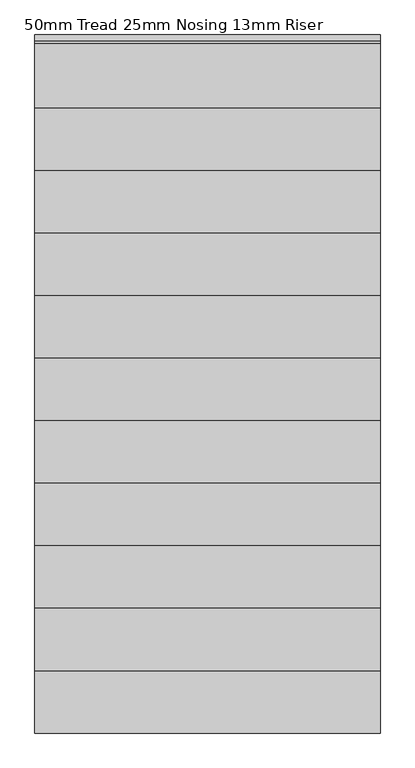
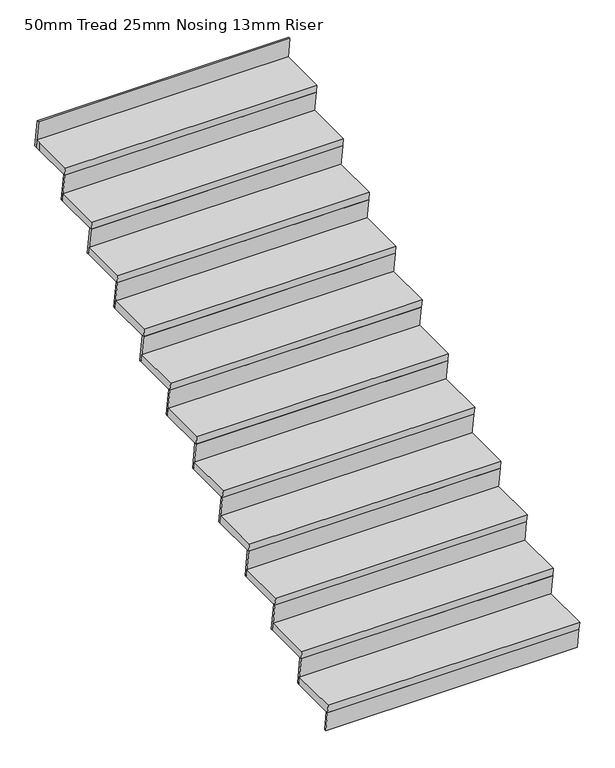
"""IFC4 building model written with IfcOpenShell, lengths in millimetres: stair flight geometry, 50mm Tread 25mm Nosing 13mm Riser."""

from ifc_helpers import new_model, si_unit, origin, place, context, project, spatial, faceted_brep, source, transform, mapped, element, save


def stair_flight_50mm_tread_25mm_nosing_13mm_riser_20ac8c47(model_context):
    return source(origin(), model_context, "Body", "Brep", [
        faceted_brep([(-499.4393676, 4584.7509075, 12676.4705882), (-499.4393676, 4591.8342409, 12626.4705882), (-2019.4393676, 4591.8342409, 12626.4705882), (-2019.4393676, 4584.7509075, 12676.4705882), (-2019.4393676, 4284.7509075, 12676.4705882), (-499.4393676, 4284.7509075, 12676.4705882), (-499.4393676, 4291.8342409, 12626.4705882), (-2019.4393676, 4291.8342409, 12626.4705882)], [[[0, 1, 2, 3]], [[3, 4, 5, 0]], [[2, 1, 6, 7]], [[4, 3, 2, 7]], [[0, 5, 6, 1]], [[5, 4, 7, 6]]]),
        faceted_brep([(-499.4393676, 4291.8342409, 12626.4705882), (-499.4393676, 4309.7509075, 12500.0), (-499.4393676, 4322.3757185, 12500.0), (-499.4393676, 4304.4590518, 12626.4705882), (-2019.4393676, 4291.8342409, 12626.4705882), (-2019.4393676, 4304.4590518, 12626.4705882), (-2019.4393676, 4322.3757185, 12500.0), (-2019.4393676, 4309.7509075, 12500.0)], [[[0, 1, 2, 3]], [[4, 5, 6, 7]], [[1, 0, 4, 7]], [[2, 1, 7, 6]], [[3, 2, 6, 5]], [[0, 3, 5, 4]]]),
        faceted_brep([(-499.4393676, 4566.8342409, 12802.9411765), (-499.4393676, 4591.8342409, 12626.4705882), (-499.4393676, 4604.4590518, 12626.4705882), (-499.4393676, 4579.4590518, 12802.9411765), (-2019.4393676, 4566.8342409, 12802.9411765), (-2019.4393676, 4579.4590518, 12802.9411765), (-2019.4393676, 4604.4590518, 12626.4705882), (-2019.4393676, 4591.8342409, 12626.4705882)], [[[0, 1, 2, 3]], [[4, 5, 6, 7]], [[1, 0, 4, 7]], [[2, 1, 7, 6]], [[3, 2, 6, 5]], [[0, 3, 5, 4]]]),
        faceted_brep([(-2019.4393676, 4859.7509075, 12852.9411765), (-2019.4393676, 4559.7509075, 12852.9411765), (-499.4393676, 4559.7509075, 12852.9411765), (-499.4393676, 4859.7509075, 12852.9411765), (-2019.4393676, 4866.8342409, 12802.9411765), (-499.4393676, 4866.8342409, 12802.9411765), (-499.4393676, 4566.8342409, 12802.9411765), (-2019.4393676, 4566.8342409, 12802.9411765)], [[[0, 1, 2, 3]], [[4, 5, 6, 7]], [[1, 0, 4, 7]], [[3, 2, 6, 5]], [[3, 5, 4, 0]], [[2, 1, 7, 6]]]),
        faceted_brep([(-499.4393676, 4841.8342409, 12979.4117647), (-499.4393676, 4866.8342409, 12802.9411765), (-499.4393676, 4879.4590518, 12802.9411765), (-499.4393676, 4854.4590518, 12979.4117647), (-2019.4393676, 4841.8342409, 12979.4117647), (-2019.4393676, 4854.4590518, 12979.4117647), (-2019.4393676, 4879.4590518, 12802.9411765), (-2019.4393676, 4866.8342409, 12802.9411765)], [[[0, 1, 2, 3]], [[4, 5, 6, 7]], [[1, 0, 4, 7]], [[2, 1, 7, 6]], [[3, 2, 6, 5]], [[0, 3, 5, 4]]]),
        faceted_brep([(-2019.4393676, 5134.7509075, 13029.4117647), (-2019.4393676, 4834.7509075, 13029.4117647), (-499.4393676, 4834.7509075, 13029.4117647), (-499.4393676, 5134.7509075, 13029.4117647), (-2019.4393676, 5141.8342409, 12979.4117647), (-499.4393676, 5141.8342409, 12979.4117647), (-499.4393676, 4841.8342409, 12979.4117647), (-2019.4393676, 4841.8342409, 12979.4117647)], [[[0, 1, 2, 3]], [[4, 5, 6, 7]], [[1, 0, 4, 7]], [[3, 2, 6, 5]], [[3, 5, 4, 0]], [[2, 1, 7, 6]]]),
        faceted_brep([(-499.4393676, 5116.8342409, 13155.8823529), (-499.4393676, 5141.8342409, 12979.4117647), (-499.4393676, 5154.4590518, 12979.4117647), (-499.4393676, 5129.4590518, 13155.8823529), (-2019.4393676, 5116.8342409, 13155.8823529), (-2019.4393676, 5129.4590518, 13155.8823529), (-2019.4393676, 5154.4590518, 12979.4117647), (-2019.4393676, 5141.8342409, 12979.4117647)], [[[0, 1, 2, 3]], [[4, 5, 6, 7]], [[1, 0, 4, 7]], [[2, 1, 7, 6]], [[3, 2, 6, 5]], [[0, 3, 5, 4]]]),
        faceted_brep([(-2019.4393676, 5409.7509075, 13205.8823529), (-2019.4393676, 5109.7509075, 13205.8823529), (-499.4393676, 5109.7509075, 13205.8823529), (-499.4393676, 5409.7509075, 13205.8823529), (-2019.4393676, 5416.8342409, 13155.8823529), (-499.4393676, 5416.8342409, 13155.8823529), (-499.4393676, 5116.8342409, 13155.8823529), (-2019.4393676, 5116.8342409, 13155.8823529)], [[[0, 1, 2, 3]], [[4, 5, 6, 7]], [[1, 0, 4, 7]], [[3, 2, 6, 5]], [[3, 5, 4, 0]], [[2, 1, 7, 6]]]),
        faceted_brep([(-499.4393676, 5391.8342409, 13332.3529412), (-499.4393676, 5416.8342409, 13155.8823529), (-499.4393676, 5429.4590518, 13155.8823529), (-499.4393676, 5404.4590518, 13332.3529412), (-2019.4393676, 5391.8342409, 13332.3529412), (-2019.4393676, 5404.4590518, 13332.3529412), (-2019.4393676, 5429.4590518, 13155.8823529), (-2019.4393676, 5416.8342409, 13155.8823529)], [[[0, 1, 2, 3]], [[4, 5, 6, 7]], [[1, 0, 4, 7]], [[2, 1, 7, 6]], [[3, 2, 6, 5]], [[0, 3, 5, 4]]]),
        faceted_brep([(-2019.4393676, 5684.7509075, 13382.3529412), (-2019.4393676, 5384.7509075, 13382.3529412), (-499.4393676, 5384.7509075, 13382.3529412), (-499.4393676, 5684.7509075, 13382.3529412), (-2019.4393676, 5691.8342409, 13332.3529412), (-499.4393676, 5691.8342409, 13332.3529412), (-499.4393676, 5391.8342409, 13332.3529412), (-2019.4393676, 5391.8342409, 13332.3529412)], [[[0, 1, 2, 3]], [[4, 5, 6, 7]], [[1, 0, 4, 7]], [[3, 2, 6, 5]], [[3, 5, 4, 0]], [[2, 1, 7, 6]]]),
        faceted_brep([(-499.4393676, 5666.8342409, 13508.8235294), (-499.4393676, 5691.8342409, 13332.3529412), (-499.4393676, 5704.4590518, 13332.3529412), (-499.4393676, 5679.4590518, 13508.8235294), (-2019.4393676, 5666.8342409, 13508.8235294), (-2019.4393676, 5679.4590518, 13508.8235294), (-2019.4393676, 5704.4590518, 13332.3529412), (-2019.4393676, 5691.8342409, 13332.3529412)], [[[0, 1, 2, 3]], [[4, 5, 6, 7]], [[1, 0, 4, 7]], [[2, 1, 7, 6]], [[3, 2, 6, 5]], [[0, 3, 5, 4]]]),
        faceted_brep([(-2019.4393676, 5959.7509075, 13558.8235294), (-2019.4393676, 5659.7509075, 13558.8235294), (-499.4393676, 5659.7509075, 13558.8235294), (-499.4393676, 5959.7509075, 13558.8235294), (-2019.4393676, 5966.8342409, 13508.8235294), (-499.4393676, 5966.8342409, 13508.8235294), (-499.4393676, 5666.8342409, 13508.8235294), (-2019.4393676, 5666.8342409, 13508.8235294)], [[[0, 1, 2, 3]], [[4, 5, 6, 7]], [[1, 0, 4, 7]], [[3, 2, 6, 5]], [[3, 5, 4, 0]], [[2, 1, 7, 6]]]),
        faceted_brep([(-499.4393676, 5941.8342409, 13685.2941176), (-499.4393676, 5966.8342409, 13508.8235294), (-499.4393676, 5979.4590518, 13508.8235294), (-499.4393676, 5954.4590518, 13685.2941176), (-2019.4393676, 5941.8342409, 13685.2941176), (-2019.4393676, 5954.4590518, 13685.2941176), (-2019.4393676, 5979.4590518, 13508.8235294), (-2019.4393676, 5966.8342409, 13508.8235294)], [[[0, 1, 2, 3]], [[4, 5, 6, 7]], [[1, 0, 4, 7]], [[2, 1, 7, 6]], [[3, 2, 6, 5]], [[0, 3, 5, 4]]]),
        faceted_brep([(-2019.4393676, 6234.7509075, 13735.2941176), (-2019.4393676, 5934.7509075, 13735.2941176), (-499.4393676, 5934.7509075, 13735.2941176), (-499.4393676, 6234.7509075, 13735.2941176), (-2019.4393676, 6241.8342409, 13685.2941176), (-499.4393676, 6241.8342409, 13685.2941176), (-499.4393676, 5941.8342409, 13685.2941176), (-2019.4393676, 5941.8342409, 13685.2941176)], [[[0, 1, 2, 3]], [[4, 5, 6, 7]], [[1, 0, 4, 7]], [[3, 2, 6, 5]], [[3, 5, 4, 0]], [[2, 1, 7, 6]]]),
        faceted_brep([(-499.4393676, 6216.8342409, 13861.7647059), (-499.4393676, 6241.8342409, 13685.2941176), (-499.4393676, 6254.4590518, 13685.2941176), (-499.4393676, 6229.4590518, 13861.7647059), (-2019.4393676, 6216.8342409, 13861.7647059), (-2019.4393676, 6229.4590518, 13861.7647059), (-2019.4393676, 6254.4590518, 13685.2941176), (-2019.4393676, 6241.8342409, 13685.2941176)], [[[0, 1, 2, 3]], [[4, 5, 6, 7]], [[1, 0, 4, 7]], [[2, 1, 7, 6]], [[3, 2, 6, 5]], [[0, 3, 5, 4]]]),
        faceted_brep([(-2019.4393676, 6509.7509075, 13911.7647059), (-2019.4393676, 6209.7509075, 13911.7647059), (-499.4393676, 6209.7509075, 13911.7647059), (-499.4393676, 6509.7509075, 13911.7647059), (-2019.4393676, 6516.8342409, 13861.7647059), (-499.4393676, 6516.8342409, 13861.7647059), (-499.4393676, 6216.8342409, 13861.7647059), (-2019.4393676, 6216.8342409, 13861.7647059)], [[[0, 1, 2, 3]], [[4, 5, 6, 7]], [[1, 0, 4, 7]], [[3, 2, 6, 5]], [[3, 5, 4, 0]], [[2, 1, 7, 6]]]),
        faceted_brep([(-499.4393676, 6491.8342409, 14038.2352941), (-499.4393676, 6516.8342409, 13861.7647059), (-499.4393676, 6529.4590518, 13861.7647059), (-499.4393676, 6504.4590518, 14038.2352941), (-2019.4393676, 6491.8342409, 14038.2352941), (-2019.4393676, 6504.4590518, 14038.2352941), (-2019.4393676, 6529.4590518, 13861.7647059), (-2019.4393676, 6516.8342409, 13861.7647059)], [[[0, 1, 2, 3]], [[4, 5, 6, 7]], [[1, 0, 4, 7]], [[2, 1, 7, 6]], [[3, 2, 6, 5]], [[0, 3, 5, 4]]]),
        faceted_brep([(-2019.4393676, 6784.7509075, 14088.2352941), (-2019.4393676, 6484.7509075, 14088.2352941), (-499.4393676, 6484.7509075, 14088.2352941), (-499.4393676, 6784.7509075, 14088.2352941), (-2019.4393676, 6791.8342409, 14038.2352941), (-499.4393676, 6791.8342409, 14038.2352941), (-499.4393676, 6491.8342409, 14038.2352941), (-2019.4393676, 6491.8342409, 14038.2352941)], [[[0, 1, 2, 3]], [[4, 5, 6, 7]], [[1, 0, 4, 7]], [[3, 2, 6, 5]], [[3, 5, 4, 0]], [[2, 1, 7, 6]]]),
        faceted_brep([(-499.4393676, 6766.8342409, 14214.7058824), (-499.4393676, 6791.8342409, 14038.2352941), (-499.4393676, 6804.4590518, 14038.2352941), (-499.4393676, 6779.4590518, 14214.7058824), (-2019.4393676, 6766.8342409, 14214.7058824), (-2019.4393676, 6779.4590518, 14214.7058824), (-2019.4393676, 6804.4590518, 14038.2352941), (-2019.4393676, 6791.8342409, 14038.2352941)], [[[0, 1, 2, 3]], [[4, 5, 6, 7]], [[1, 0, 4, 7]], [[2, 1, 7, 6]], [[3, 2, 6, 5]], [[0, 3, 5, 4]]]),
        faceted_brep([(-2019.4393676, 7059.7509075, 14264.7058824), (-2019.4393676, 6759.7509075, 14264.7058824), (-499.4393676, 6759.7509075, 14264.7058824), (-499.4393676, 7059.7509075, 14264.7058824), (-2019.4393676, 7066.8342409, 14214.7058824), (-499.4393676, 7066.8342409, 14214.7058824), (-499.4393676, 6766.8342409, 14214.7058824), (-2019.4393676, 6766.8342409, 14214.7058824)], [[[0, 1, 2, 3]], [[4, 5, 6, 7]], [[1, 0, 4, 7]], [[3, 2, 6, 5]], [[3, 5, 4, 0]], [[2, 1, 7, 6]]]),
        faceted_brep([(-499.4393676, 7316.8342409, 14567.6470588), (-499.4393676, 7341.8342409, 14391.1764706), (-499.4393676, 7354.4590518, 14391.1764706), (-499.4393676, 7329.4590518, 14567.6470588), (-2019.4393676, 7316.8342409, 14567.6470588), (-2019.4393676, 7329.4590518, 14567.6470588), (-2019.4393676, 7354.4590518, 14391.1764706), (-2019.4393676, 7341.8342409, 14391.1764706)], [[[0, 1, 2, 3]], [[4, 5, 6, 7]], [[1, 0, 4, 7]], [[2, 1, 7, 6]], [[3, 2, 6, 5]], [[0, 3, 5, 4]]]),
        faceted_brep([(-499.4393676, 7041.8342409, 14391.1764706), (-499.4393676, 7066.8342409, 14214.7058824), (-499.4393676, 7079.4590518, 14214.7058824), (-499.4393676, 7054.4590518, 14391.1764706), (-2019.4393676, 7041.8342409, 14391.1764706), (-2019.4393676, 7054.4590518, 14391.1764706), (-2019.4393676, 7079.4590518, 14214.7058824), (-2019.4393676, 7066.8342409, 14214.7058824)], [[[0, 1, 2, 3]], [[4, 5, 6, 7]], [[1, 0, 4, 7]], [[2, 1, 7, 6]], [[3, 2, 6, 5]], [[0, 3, 5, 4]]]),
        faceted_brep([(-2019.4393676, 7334.7509075, 14441.1764706), (-2019.4393676, 7309.7509075, 14441.1764706), (-2019.4393676, 7034.7509075, 14441.1764706), (-499.4393676, 7034.7509075, 14441.1764706), (-499.4393676, 7334.7509075, 14441.1764706), (-2019.4393676, 7341.8342409, 14391.1764706), (-499.4393676, 7341.8342409, 14391.1764706), (-499.4393676, 7041.8342409, 14391.1764706), (-2019.4393676, 7041.8342409, 14391.1764706), (-2019.4393676, 7309.7509075, 14391.1764706)], [[[0, 1, 2, 3, 4]], [[5, 6, 7, 8, 9]], [[1, 0, 5, 9]], [[2, 1, 9, 8]], [[4, 3, 7, 6]], [[4, 6, 5, 0]], [[3, 2, 8, 7]]]),
    ])


if __name__ == "__main__":
    model = new_model("IFC4")
    model_context = context("Model", 3, world=origin())
    ifc_project = project(units=[si_unit("LENGTHUNIT", "METRE", prefix="MILLI")], contexts=[model_context])
    site = spatial("IfcSite", under=ifc_project)
    building = spatial("IfcBuilding", under=site)
    placement = place(None, origin())
    stair_flight_50mm_tread_25mm_nosing_13mm_riser_shape = stair_flight_50mm_tread_25mm_nosing_13mm_riser_20ac8c47(model_context)
    element("IfcStairFlight", 1, ObjectType="50mm Tread 25mm Nosing 13mm Riser", at=placement, inside=building, context=model_context, shape_type="MappedRepresentation", body=[
        mapped(stair_flight_50mm_tread_25mm_nosing_13mm_riser_shape, transform((0.0, 0.0, 0.0), x_axis=(1.0, 0.0, 0.0), y_axis=(0.0, 1.0, 0.0), z_axis=(0.0, 0.0, 1.0))),
    ])
    save(model, "model.ifc")
